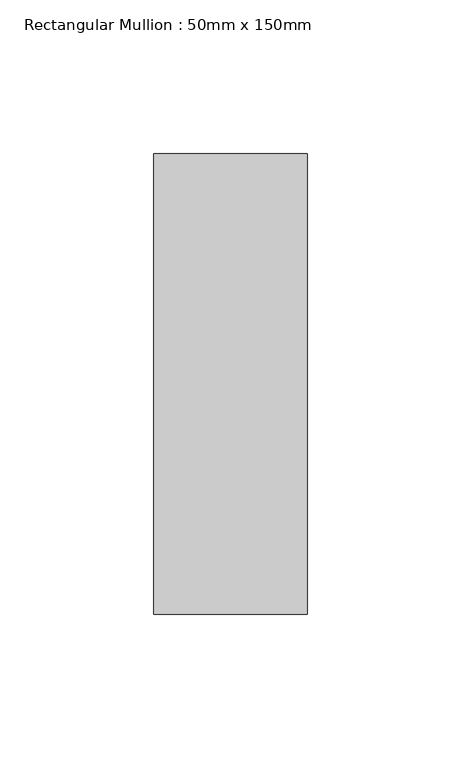
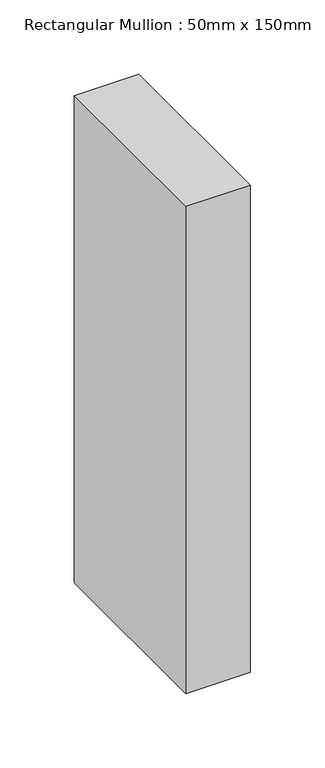
"""IFC4 building model written with IfcOpenShell, lengths in millimetres: member geometry, Rectangular Mullion : 50mm x 150mm."""

from ifc_helpers import new_model, si_unit, frame, origin, place, context, project, spatial, polyline, outline, extrude, source, transform, mapped, element, save


def rectangular_mullion_50mm_x_150mm_e11a3e7b(model_context):
    return source(origin(), model_context, "Body", "SweptSolid", [
        extrude(outline(polyline([(0.0, 75.0), (0.0, -75.0), (-50.0, -75.0), (-50.0, 75.0), (0.0, 75.0)])), frame((0.0, 0.0, -400.0), z_axis=(0.0, 0.0, 1.0), x_axis=(1.0, 0.0, 0.0)), (0.0, 0.0, 1.0), 400.0),
    ])


if __name__ == "__main__":
    model = new_model("IFC4")
    model_context = context("Model", 3, world=origin())
    ifc_project = project(units=[si_unit("LENGTHUNIT", "METRE", prefix="MILLI")], contexts=[model_context])
    site = spatial("IfcSite", under=ifc_project)
    building = spatial("IfcBuilding", under=site)
    placement = place(None, origin())
    rectangular_mullion_50mm_x_150mm_shape = rectangular_mullion_50mm_x_150mm_e11a3e7b(model_context)
    element("IfcMember", 1, ObjectType="Rectangular Mullion : 50mm x 150mm", at=placement, inside=building, context=model_context, shape_type="MappedRepresentation", body=[
        mapped(rectangular_mullion_50mm_x_150mm_shape, transform((0.0, 0.0, 0.0), x_axis=(1.0, 0.0, 0.0), y_axis=(0.0, 1.0, 0.0), z_axis=(0.0, 0.0, 1.0))),
    ])
    save(model, "model.ifc")

# Revit data of these elements
# Type "Rectangular Mullion : 50mm x 150mm"
#   built-in parameter 1007304 = 0.492126 (stored number, unit not read)
#   built-in parameter 1007301 = 0.082021 (stored number, unit not read)
#   built-in parameter 1007300 = 0.082021 (stored number, unit not read)
# Element 1 (IfcMember, "Rectangular Mullion : 50mm x 150mm")
#   Materials on its faces: "Aluminum"
# Materials
#   "Aluminum": class "Metal", colour RGB 244 244 244, transparency 0, Description = "Aluminum 6061", Cost = 0
